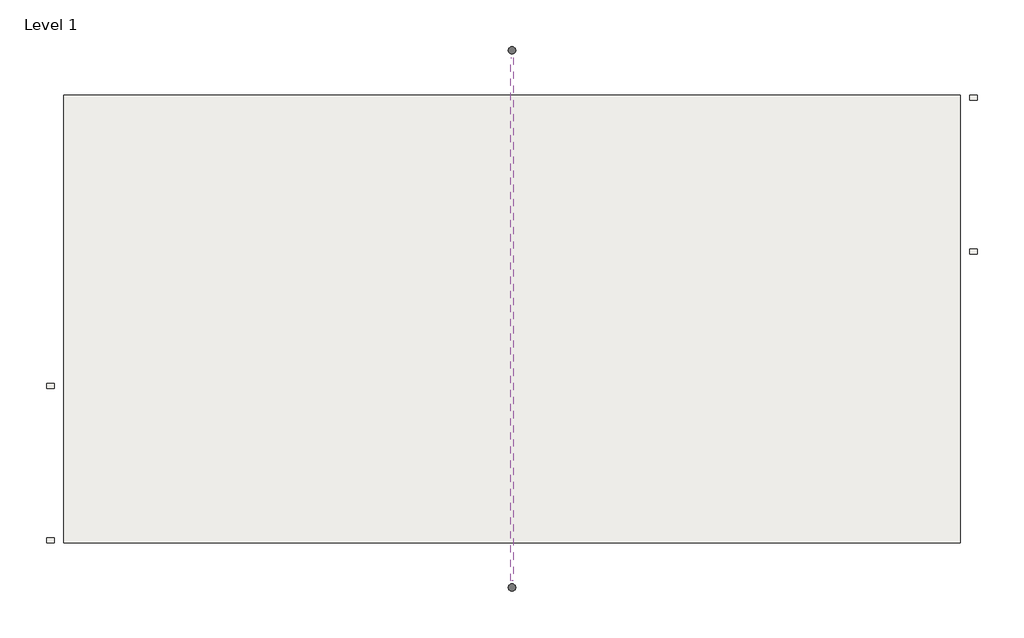
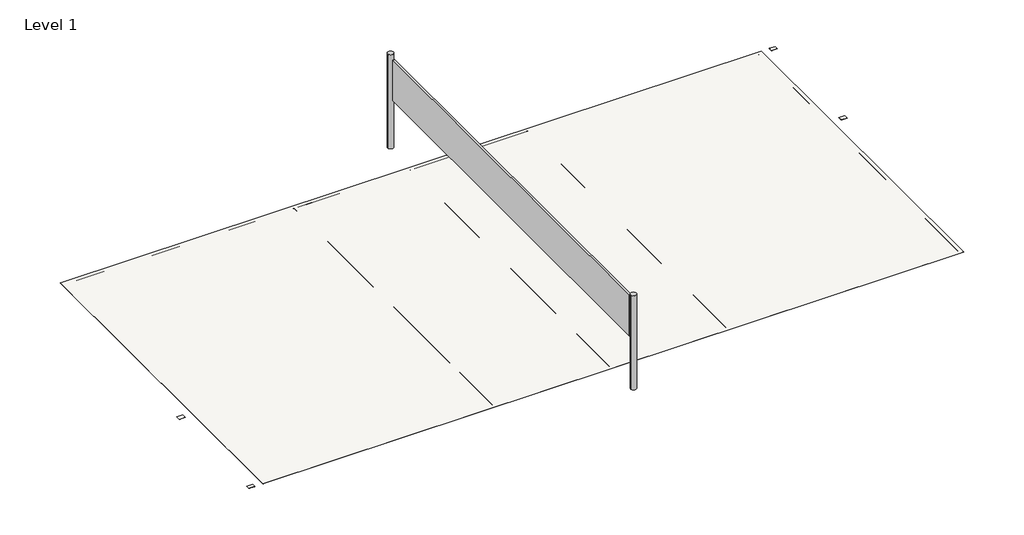
# One storey: 3 proxies, 2 slabs.
"""IFC4 building model written with IfcOpenShell, lengths in millimetres."""

from ifc_helpers import new_model, si_unit, point, frame, frame_2d, origin, origin_with_axes, place, context, project, spatial, polyline, circle_curve, trimmed, segment, composite_curve, outline, extrude, element, save

model = new_model("IFC4")

# Units and contexts
model_context = context("Model", 3, world=origin())
ifc_project = project(units=[si_unit("LENGTHUNIT", "METRE", prefix="MILLI")], contexts=[model_context])

# Site, building, storey
site = spatial("IfcSite", under=ifc_project)
building = spatial("IfcBuilding", under=site)
storey = spatial("IfcBuildingStorey", under=building, Name="Level 1", Elevation=0.0)

# Proxies
placement = place(None, origin())
element("IfcBuildingElementProxy", 1, Name="Mass 1 : Mass 1", ObjectType="Mass 1 : Mass 1", at=placement, inside=storey, context=model_context, shape_type="SweptSolid", body=[
    extrude(outline(composite_curve([segment(trimmed(circle_curve(frame_2d((15029.159193, 5689.393458)), 76.2), [point((14952.959193, 5689.393458))], [point((15105.359193, 5689.393458))], False, "CARTESIAN"), True, "CONTINUOUS"), segment(trimmed(circle_curve(frame_2d((15029.159193, 5689.393458)), 76.2), [point((15105.359193, 5689.393458))], [point((14952.959193, 5689.393458))], False, "CARTESIAN"), True, "CONTINUOUS")], self_intersect=False)), origin_with_axes(), (0.0, 0.0, 1.0), 2590.8),
])
element("IfcBuildingElementProxy", 2, Name="Mass 2 : Mass 1", ObjectType="Mass 2 : Mass 1", at=placement, inside=storey, context=model_context, shape_type="SweptSolid", body=[
    extrude(outline(composite_curve([segment(trimmed(circle_curve(frame_2d((15029.159193, 16662.193458)), 76.2), [point((14952.959193, 16662.193458))], [point((15105.359193, 16662.193458))], False, "CARTESIAN"), True, "CONTINUOUS"), segment(trimmed(circle_curve(frame_2d((15029.159193, 16662.193458)), 76.2), [point((15105.359193, 16662.193458))], [point((14952.959193, 16662.193458))], False, "CARTESIAN"), True, "CONTINUOUS")], self_intersect=False)), origin_with_axes(), (0.0, 0.0, 1.0), 2590.8),
])
element("IfcBuildingElementProxy", 3, Name="Mass 3 : Mass 3", ObjectType="Mass 3 : Mass 3", at=placement, inside=storey, context=model_context, shape_type="SweptSolid", body=[
    extrude(outline(polyline([(15003.759193, 16513.9879466), (15054.559193, 16513.9879466), (15054.559193, 5824.4489036), (15003.759193, 5824.4489036), (15003.759193, 16513.9879466)])), frame((0.0, 0.0, 1370.6596256), z_axis=(0.0, 0.0, 1.0), x_axis=(1.0, 0.0, 0.0)), (0.0, 0.0, 1.0), 1121.43554),
])

# Slabs
element("IfcSlab", 4, ObjectType="Concrete", at=placement, inside=storey, context=model_context, shape_type="SweptSolid", body=[
    extrude(outline(polyline([(24173.159193, 6603.793458), (5885.159193, 6603.793458), (5885.159193, 15747.793458), (24173.159193, 15747.793458), (24173.159193, 6603.793458)])), frame((0.0, 0.0, -1.5875), z_axis=(0.0, 0.0, 1.0), x_axis=(1.0, 0.0, 0.0)), (0.0, 0.0, 1.0), 1.5875),
])
element("IfcSlab", 5, ObjectType="Paint", at=placement, inside=storey, context=model_context, shape_type="SweptSolid", body=[
    extrude(outline(polyline([(5885.159193, 15747.793458), (24173.159193, 15747.793458), (24173.159193, 6603.793458), (5885.159193, 6603.793458), (5885.159193, 15747.793458)]), holes=[polyline([(5986.759193, 15646.193458), (5986.759193, 6705.393458), (11930.359193, 6705.393458), (11930.359193, 15646.193458), (5986.759193, 15646.193458)]), polyline([(14978.359193, 6705.393458), (14978.359193, 15646.193458), (12031.959193, 15646.193458), (12031.959193, 6705.393458), (14978.359193, 6705.393458)]), polyline([(24071.559193, 15646.193458), (18127.959193, 15646.193458), (18127.959193, 6705.393458), (24071.559193, 6705.393458), (24071.559193, 15646.193458)]), polyline([(18026.359193, 15646.193458), (15079.959193, 15646.193458), (15079.959193, 6705.393458), (18026.359193, 6705.393458), (18026.359193, 15646.193458)])]), frame((0.0, 0.0, -1.5875), z_axis=(0.0, 0.0, 1.0), x_axis=(1.0, 0.0, 0.0)), (0.0, 0.0, 1.0), 1.5875),
    extrude(outline(polyline([(24376.359193, 15747.793458), (24528.759193, 15747.793458), (24528.759193, 15646.193458), (24376.359193, 15646.193458), (24376.359193, 15747.793458)])), frame((0.0, 0.0, -1.5875), z_axis=(0.0, 0.0, 1.0), x_axis=(1.0, 0.0, 0.0)), (0.0, 0.0, 1.0), 1.5875),
    extrude(outline(polyline([(24376.359193, 12598.193458), (24528.759193, 12598.193458), (24528.759193, 12496.593458), (24376.359193, 12496.593458), (24376.359193, 12598.193458)])), frame((0.0, 0.0, -1.5875), z_axis=(0.0, 0.0, 1.0), x_axis=(1.0, 0.0, 0.0)), (0.0, 0.0, 1.0), 1.5875),
    extrude(outline(polyline([(5681.959193, 9854.993458), (5681.959193, 9753.393458), (5529.559193, 9753.393458), (5529.559193, 9854.993458), (5681.959193, 9854.993458)])), frame((0.0, 0.0, -1.5875), z_axis=(0.0, 0.0, 1.0), x_axis=(1.0, 0.0, 0.0)), (0.0, 0.0, 1.0), 1.5875),
    extrude(outline(polyline([(5681.959193, 6705.393458), (5681.959193, 6603.793458), (5529.559193, 6603.793458), (5529.559193, 6705.393458), (5681.959193, 6705.393458)])), frame((0.0, 0.0, -1.5875), z_axis=(0.0, 0.0, 1.0), x_axis=(1.0, 0.0, 0.0)), (0.0, 0.0, 1.0), 1.5875),
])

save(model, "model.ifc")

# Revit data of these elements
# Project information
#   Project Issue Date = "Issue Date"
#   Project Status = "Project Status"
#   Client Name = "Owner"
#   Project Address = "Enter address here"
#   Project Name = "PROJECT NAME"
#   Project Number = "Project Number"
# Type "Concrete"
#   Assembly Code = "B1010"
#   Thickness = 0' - 0 1/16"
#   Function = 0
#   Layers, outside or top first: 0' - 0 1/16" "Concrete, Precast" (function 1)
# Type "Paint"
#   Assembly Code = "B1010"
#   Thickness = 0' - 0 1/16"
#   Function = 0
#   Layers, outside or top first: 0' - 0 1/16" "Paint-Philips-White" (function 1)
# Element 1 (IfcBuildingElementProxy, "Mass 1 : Mass 1")
#   Phase Created = New Construction
#   Materials on its faces: "Default Form"
# Element 2 (IfcBuildingElementProxy, "Mass 2 : Mass 1")
#   Phase Created = New Construction
#   Materials on its faces: "Default Form"
# Element 3 (IfcBuildingElementProxy, "Mass 3 : Mass 3")
#   Phase Created = New Construction
#   Materials on its faces: "Default Form"
# Element 4 (IfcSlab, "Concrete")
#   Height Offset From Level = 0' - 0"
#   Phase Created = New Construction
#   Materials on its faces: "Concrete, Precast"
# Element 5 (IfcSlab, "Paint")
#   built-in parameter 1001955 = 3.14159 (stored number, unit not read)
#   Height Offset From Level = 0' - 0"
#   Phase Created = New Construction
#   Materials on its faces: "Paint-Philips-White"
# Materials
#   "Concrete, Precast": class "Concrete", colour RGB 115 116 108, transparency 0, Description = "Precast concrete", Cost = 0
#   "Paint-Philips-White": class "Paint", colour RGB 255 255 255, transparency 0
#   "Default Form": class "Generic", colour RGB 185 189 196, transparency 0.49, Cost = 0
